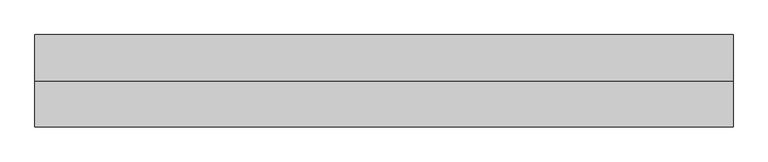
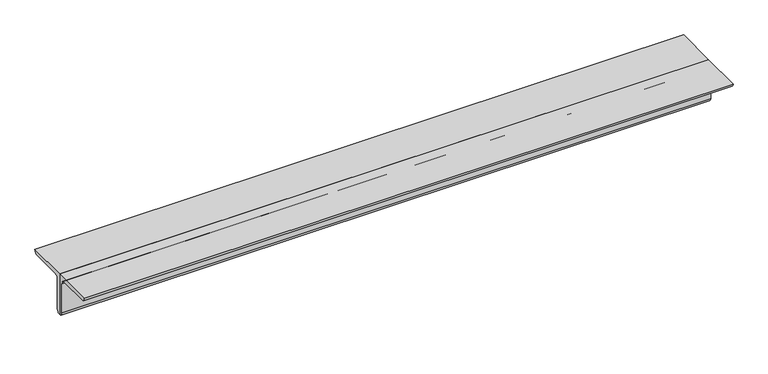
"""IFC4 building model written with IfcOpenShell, lengths in millimetres: member geometry, 0123_Steel Framing_2Ls-KSD3502 : H_SB_AR_S04_2Ls-130x130x12_VBR1."""

from ifc_helpers import new_model, si_unit, point, frame, frame_2d, origin, place, context, project, spatial, polyline, circle_curve, trimmed, segment, composite_curve, outline, extrude, source, transform, mapped, element, save


def member_d0207f13(model_context):
    return source(origin(), model_context, "Body", "SweptSolid", [
        extrude(outline(composite_curve([segment(polyline([(0.0, 36.4), (130.0, 36.4)]), True, "CONTINUOUS"), segment(trimmed(circle_curve(frame_2d((118.0, 36.4)), 12.0), [point((130.0, 36.4))], [point((118.0, 24.4))], False, "CARTESIAN"), True, "CONTINUOUS"), segment(polyline([(118.0, 24.4), (24.0, 24.4)]), True, "CONTINUOUS"), segment(trimmed(circle_curve(frame_2d((24.0, 12.4)), 12.0), [point((24.0, 24.4))], [point((12.0, 12.4))], True, "CARTESIAN"), True, "CONTINUOUS"), segment(polyline([(12.0, 12.4), (12.0, -81.6)]), True, "CONTINUOUS"), segment(trimmed(circle_curve(frame_2d((0.0, -81.6)), 12.0), [point((12.0, -81.6))], [point((0.0, -93.6))], False, "CARTESIAN"), True, "CONTINUOUS"), segment(polyline([(0.0, -93.6), (0.0, 36.4)]), True, "CONTINUOUS")], self_intersect=False)), frame((-1052.8208184, 0.0, 0.0), z_axis=(1.0, 0.0, 0.0), x_axis=(0.0, 1.0, 0.0)), (0.0, 0.0, 1.0), 1965.6424176),
        extrude(outline(composite_curve([segment(polyline([(0.0, 36.4), (0.0, -93.6)]), True, "CONTINUOUS"), segment(trimmed(circle_curve(frame_2d((0.0, -81.6)), 12.0), [point((0.0, -93.6))], [point((-12.0, -81.6))], False, "CARTESIAN"), True, "CONTINUOUS"), segment(polyline([(-12.0, -81.6), (-12.0, 12.4)]), True, "CONTINUOUS"), segment(trimmed(circle_curve(frame_2d((-24.0, 12.4)), 12.0), [point((-12.0, 12.4))], [point((-24.0, 24.4))], True, "CARTESIAN"), True, "CONTINUOUS"), segment(polyline([(-24.0, 24.4), (-118.0, 24.4)]), True, "CONTINUOUS"), segment(trimmed(circle_curve(frame_2d((-118.0, 36.4)), 12.0), [point((-118.0, 24.4))], [point((-130.0, 36.4))], False, "CARTESIAN"), True, "CONTINUOUS"), segment(polyline([(-130.0, 36.4), (0.0, 36.4)]), True, "CONTINUOUS")], self_intersect=False)), frame((-1052.8208184, 0.0, 0.0), z_axis=(1.0, 0.0, 0.0), x_axis=(0.0, 1.0, 0.0)), (0.0, 0.0, 1.0), 1965.6424176),
    ])


if __name__ == "__main__":
    model = new_model("IFC4")
    model_context = context("Model", 3, world=origin())
    ifc_project = project(units=[si_unit("LENGTHUNIT", "METRE", prefix="MILLI")], contexts=[model_context])
    site = spatial("IfcSite", under=ifc_project)
    building = spatial("IfcBuilding", under=site)
    placement = place(None, origin())
    member_shape = member_d0207f13(model_context)
    element("IfcMember", 1, ObjectType="0123_Steel Framing_2Ls-KSD3502 : H_SB_AR_S04_2Ls-130x130x12_VBR1", at=placement, inside=building, context=model_context, shape_type="MappedRepresentation", body=[
        mapped(member_shape, transform((0.0, 0.0, 0.0), x_axis=(1.0, 0.0, 0.0), y_axis=(0.0, 1.0, 0.0), z_axis=(0.0, 0.0, 1.0))),
    ])
    save(model, "model.ifc")

# Revit data of these elements
# Type "0123_Steel Framing_2Ls-KSD3502 : H_SB_AR_S04_2Ls-130x130x12_VBR1"
#   Assembly Code = "B10"
#   Legs = "SLBB"
#   W = 8.97
#   Perimeter = 1.04 m²/m
#   Nominal Weight = 46.80 kgf/m
#   Length [instance default] = 1000 mm
#   Space = 0 mm
#   b = 130 mm
#   d = 130 mm
#   t = 12 mm
#   y = 36.4 mm
#   A = 0.005952 m²
#   Structural Material [instance default] = Steel ASTM A36
# Element 1 (IfcMember, "0123_Steel Framing_2Ls-KSD3502 : H_SB_AR_S04_2Ls-130x130x12_VBR1")
#   Structural Material = Steel, 45-345
#   Materials on its faces: "Steel, 45-345"
# Materials
#   "Steel ASTM A36": class "Metal", colour RGB 199 199 199, transparency 0, Description = "Structural steel, ASTM A36 Grade B, mill finish", Cost = 0
#   "Steel, 45-345": class "Metal", colour RGB 189 187 185, transparency 0, Description = "Steel 345 MPa", Cost = 0
